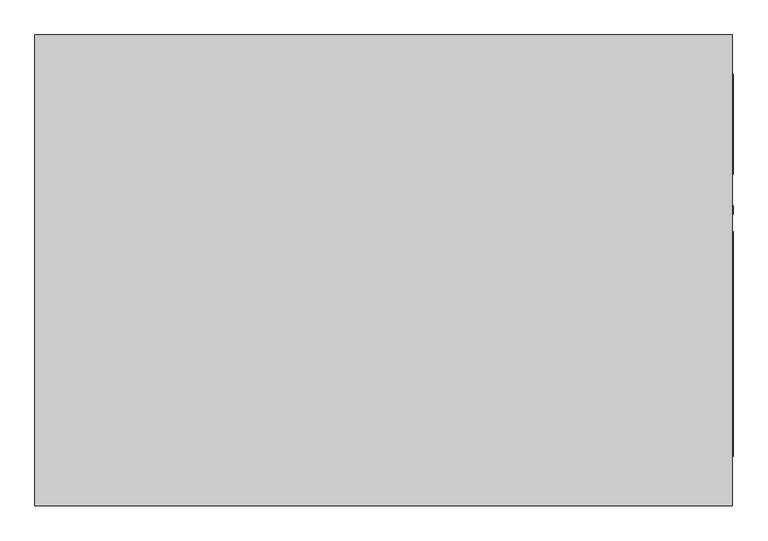
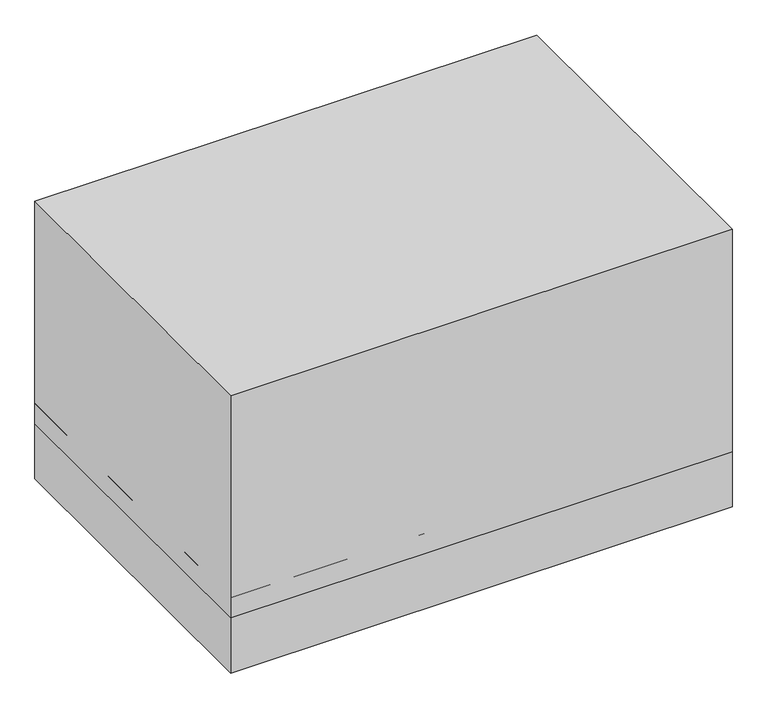
"""IFC4 building model written with IfcOpenShell, lengths in millimetres: proxy geometry, Carrier_48TC_Standard_Efficiency_Gas_Heat_Electric_Cooling_Packaged_Rooftop_Unit_3_to_15_nominal_tons : 7.5 ton 48TC**08."""

from ifc_helpers import new_model, si_unit, point, frame, frame_2d, origin, origin_with_axes, place, context, project, spatial, polyline, circle_curve, trimmed, segment, composite_curve, outline, extrude, source, transform, mapped, element, save
from ifc_brep_helpers import plane_surface, revolved_surface, advanced_brep


def mechanical_equipment_22992897(model_context):
    return source(origin(), model_context, "Body", "SolidModel", [
        extrude(outline(composite_curve([segment(trimmed(circle_curve(frame_2d((193.675, 438.15)), 13.2953125), [point((180.3796875, 438.15))], [point((206.9703125, 438.15))], False, "CARTESIAN"), True, "CONTINUOUS"), segment(trimmed(circle_curve(frame_2d((193.675, 438.15)), 13.2953125), [point((206.9703125, 438.15))], [point((180.3796875, 438.15))], False, "CARTESIAN"), True, "CONTINUOUS")], self_intersect=False)), frame((1119.1875, 0.0, 0.0), z_axis=(1.0, 0.0, 0.0), x_axis=(0.0, 1.0, 0.0)), (0.0, 0.0, 1.0), 3.175),
        advanced_brep(
        [(1119.1875, 755.65, 1308.1), (-1119.1875, 755.65, 1308.1), (-1119.1875, -755.65, 1308.1), (1119.1875, -755.65, 1308.1), (1119.1875, 755.65, 260.35), (1119.1875, -755.65, 260.35), (-1119.1875, -755.65, 260.35), (-1119.1875, 755.65, 260.35), (1036.6375, -596.9, 260.35), (1036.6375, 0.0, 260.35), (681.0375, 0.0, 260.35), (681.0375, -596.9, 260.35), (1036.6375, 590.55, 260.35), (112.7125, 590.55, 260.35), (112.7125, 269.875, 260.35), (1036.6375, 269.875, 260.35), (176.8078125, -107.95, 260.35), (150.2171875, -107.95, 260.35), (-355.6, -476.25, 260.35), (-377.825, -476.25, 260.35), (-344.4875, -349.25, 260.35), (-388.9375, -349.25, 260.35), (-344.4875, -298.45, 260.35), (-388.9375, -298.45, 260.35), (1036.6375, -596.9, 381.0), (681.0375, -596.9, 381.0), (681.0375, 0.0, 381.0), (1036.6375, 0.0, 381.0), (1036.6375, 590.55, 381.0), (1036.6375, 269.875, 381.0), (112.7125, 269.875, 381.0), (112.7125, 590.55, 381.0), (176.8078125, -107.95, 406.4), (150.2171875, -107.95, 406.4), (-355.6, -476.25, 406.4), (-377.825, -476.25, 406.4), (-344.4875, -349.25, 406.4), (-388.9375, -349.25, 406.4), (-344.4875, -298.45, 406.4), (-388.9375, -298.45, 406.4)],
        [
            (0, 1),
            (1, 2),
            (2, 3),
            (3, 0),
            (4, 5),
            (5, 6),
            (6, 7),
            (7, 4),
            (8, 9),
            (9, 10),
            (10, 11),
            (11, 8),
            (12, 13),
            (13, 14),
            (14, 15),
            (15, 12),
            (16, 17, circle_curve(frame((163.5125, -107.95, 260.35), z_axis=(0.0, 0.0, 1.0), x_axis=(-1.0, 0.0, 0.0)), 13.2953125)),
            (17, 16, circle_curve(frame((163.5125, -107.95, 260.35), z_axis=(0.0, 0.0, 1.0), x_axis=(-1.0, 0.0, 0.0)), 13.2953125)),
            (18, 19, circle_curve(frame((-366.7125, -476.25, 260.35), z_axis=(0.0, 0.0, 1.0), x_axis=(-1.0, 0.0, 0.0)), 11.1125)),
            (19, 18, circle_curve(frame((-366.7125, -476.25, 260.35), z_axis=(0.0, 0.0, 1.0), x_axis=(-1.0, 0.0, 0.0)), 11.1125)),
            (20, 21, circle_curve(frame((-366.7125, -349.25, 260.35), z_axis=(0.0, 0.0, 1.0), x_axis=(-1.0, 0.0, 0.0)), 22.225)),
            (21, 20, circle_curve(frame((-366.7125, -349.25, 260.35), z_axis=(0.0, 0.0, 1.0), x_axis=(-1.0, 0.0, 0.0)), 22.225)),
            (22, 23, circle_curve(frame((-366.7125, -298.45, 260.35), z_axis=(0.0, 0.0, 1.0), x_axis=(-1.0, 0.0, 0.0)), 22.225)),
            (23, 22, circle_curve(frame((-366.7125, -298.45, 260.35), z_axis=(0.0, 0.0, 1.0), x_axis=(-1.0, 0.0, 0.0)), 22.225)),
            (0, 4),
            (7, 1),
            (6, 2),
            (5, 3),
            (24, 25),
            (25, 26),
            (26, 27),
            (27, 24),
            (27, 9),
            (8, 24),
            (26, 10),
            (25, 11),
            (28, 29),
            (29, 30),
            (30, 31),
            (31, 28),
            (31, 13),
            (12, 28),
            (30, 14),
            (29, 15),
            (32, 33, circle_curve(frame((163.5125, -107.95, 406.4), z_axis=(0.0, 0.0, -1.0), x_axis=(-1.0, 0.0, 0.0)), 13.2953125)),
            (33, 32, circle_curve(frame((163.5125, -107.95, 406.4), z_axis=(0.0, 0.0, -1.0), x_axis=(-1.0, 0.0, 0.0)), 13.2953125)),
            (33, 17),
            (16, 32),
            (34, 35, circle_curve(frame((-366.7125, -476.25, 406.4), z_axis=(0.0, 0.0, -1.0), x_axis=(-1.0, 0.0, 0.0)), 11.1125)),
            (35, 34, circle_curve(frame((-366.7125, -476.25, 406.4), z_axis=(0.0, 0.0, -1.0), x_axis=(-1.0, 0.0, 0.0)), 11.1125)),
            (35, 19),
            (18, 34),
            (36, 37, circle_curve(frame((-366.7125, -349.25, 406.4), z_axis=(0.0, 0.0, -1.0), x_axis=(-1.0, 0.0, 0.0)), 22.225)),
            (37, 36, circle_curve(frame((-366.7125, -349.25, 406.4), z_axis=(0.0, 0.0, -1.0), x_axis=(-1.0, 0.0, 0.0)), 22.225)),
            (37, 21),
            (20, 36),
            (38, 39, circle_curve(frame((-366.7125, -298.45, 406.4), z_axis=(0.0, 0.0, -1.0), x_axis=(-1.0, 0.0, 0.0)), 22.225)),
            (39, 38, circle_curve(frame((-366.7125, -298.45, 406.4), z_axis=(0.0, 0.0, -1.0), x_axis=(-1.0, 0.0, 0.0)), 22.225)),
            (39, 23),
            (22, 38),
        ],
        [
            plane_surface(frame((-1119.1875, 755.65, 1308.1), z_axis=(0.0, 0.0, 1.0), x_axis=(-1.0, 0.0, 0.0))),
            plane_surface(frame((-1119.1875, 755.65, 260.35), z_axis=(0.0, 0.0, -1.0), x_axis=(1.0, 0.0, 0.0))),
            plane_surface(frame((1119.1875, 755.65, 1308.1), z_axis=(0.0, 1.0, 0.0), x_axis=(0.0, 0.0, -1.0))),
            plane_surface(frame((-1119.1875, 755.65, 1308.1), z_axis=(-1.0, 0.0, 0.0), x_axis=(0.0, 0.0, -1.0))),
            plane_surface(frame((-1119.1875, -755.65, 1308.1), z_axis=(0.0, -1.0, 0.0), x_axis=(0.0, 0.0, -1.0))),
            plane_surface(frame((1119.1875, -755.65, 1308.1), z_axis=(1.0, 0.0, 0.0), x_axis=(0.0, 0.0, -1.0))),
            plane_surface(frame((1036.6375, -596.9, 381.0), z_axis=(0.0, 0.0, -1.0), x_axis=(0.0, 1.0, 0.0))),
            plane_surface(frame((1036.6375, -596.9, 381.0), z_axis=(-1.0, 0.0, 0.0), x_axis=(0.0, 0.0, -1.0))),
            plane_surface(frame((1036.6375, 0.0, 381.0), z_axis=(0.0, -1.0, 0.0), x_axis=(0.0, 0.0, -1.0))),
            plane_surface(frame((681.0375, 0.0, 381.0), z_axis=(1.0, 0.0, 0.0), x_axis=(0.0, 0.0, -1.0))),
            plane_surface(frame((681.0375, -596.9, 381.0), z_axis=(0.0, 1.0, 0.0), x_axis=(0.0, 0.0, -1.0))),
            plane_surface(frame((112.7125, 590.55, 381.0), z_axis=(0.0, 0.0, -1.0), x_axis=(-1.0, 0.0, 0.0))),
            plane_surface(frame((1036.6375, 590.55, 381.0), z_axis=(0.0, -1.0, 0.0), x_axis=(0.0, 0.0, -1.0))),
            plane_surface(frame((112.7125, 590.55, 381.0), z_axis=(1.0, 0.0, 0.0), x_axis=(0.0, 0.0, -1.0))),
            plane_surface(frame((112.7125, 269.875, 381.0), z_axis=(0.0, 1.0, 0.0), x_axis=(0.0, 0.0, -1.0))),
            plane_surface(frame((1036.6375, 269.875, 381.0), z_axis=(-1.0, 0.0, 0.0), x_axis=(0.0, 0.0, -1.0))),
            plane_surface(frame((150.2171875, -107.95, 406.4), z_axis=(0.0, 0.0, -1.0), x_axis=(0.0, -1.0, 0.0))),
            revolved_surface(polyline([(150.2171875, -107.95, 406.4), (150.2171875, -107.95, 260.35)]), (163.5125, -107.95, 0.0), (0.0, 0.0, 1.0)),
            plane_surface(frame((-377.825, -476.25, 406.4), z_axis=(0.0, 0.0, -1.0), x_axis=(0.0, -1.0, 0.0))),
            revolved_surface(polyline([(-377.825, -476.25, 406.4), (-377.825, -476.25, 260.35)]), (-366.7125, -476.25, 0.0), (0.0, 0.0, 1.0)),
            plane_surface(frame((-388.9375, -349.25, 406.4), z_axis=(0.0, 0.0, -1.0), x_axis=(0.0, -1.0, 0.0))),
            revolved_surface(polyline([(-388.9375, -349.25, 406.4), (-388.9375, -349.25, 260.35)]), (-366.7125, -349.25, 0.0), (0.0, 0.0, 1.0)),
            plane_surface(frame((-388.9375, -298.45, 406.4), z_axis=(0.0, 0.0, -1.0), x_axis=(0.0, -1.0, 0.0))),
            revolved_surface(polyline([(-388.9375, -298.45, 406.4), (-388.9375, -298.45, 260.35)]), (-366.7125, -298.45, 0.0), (0.0, 0.0, 1.0)),
        ],
        [
            (0, [[1, 2, 3, 4]]),
            (1, [[5, 6, 7, 8], [9, 10, 11, 12], [13, 14, 15, 16], [17, 18], [19, 20], [21, 22], [23, 24]]),
            (2, [[-1, 25, -8, 26]]),
            (3, [[-2, -26, -7, 27]]),
            (4, [[-3, -27, -6, 28]]),
            (5, [[-4, -28, -5, -25]]),
            (6, [[29, 30, 31, 32]]),
            (7, [[-32, 33, -9, 34]]),
            (8, [[-31, 35, -10, -33]]),
            (9, [[-30, 36, -11, -35]]),
            (10, [[-29, -34, -12, -36]]),
            (11, [[37, 38, 39, 40]]),
            (12, [[-40, 41, -13, 42]]),
            (13, [[-39, 43, -14, -41]]),
            (14, [[-38, 44, -15, -43]]),
            (15, [[-37, -42, -16, -44]]),
            (16, [[45, 46]]),
            (17, [[-46, 47, -17, 48]]),
            (17, [[-45, -48, -18, -47]]),
            (18, [[49, 50]]),
            (19, [[-50, 51, -19, 52]]),
            (19, [[-49, -52, -20, -51]]),
            (20, [[53, 54]]),
            (21, [[-54, 55, -21, 56]]),
            (21, [[-53, -56, -22, -55]]),
            (22, [[57, 58]]),
            (23, [[-58, 59, -23, 60]]),
            (23, [[-57, -60, -24, -59]]),
        ],
    ),
        extrude(outline(polyline([(1119.1875, 755.65), (1119.1875, -755.65), (-1119.1875, -755.65), (-1119.1875, 755.65), (1119.1875, 755.65)]), holes=[polyline([(1036.6375, 590.55), (112.7125, 590.55), (112.7125, 269.875), (1036.6375, 269.875), (1036.6375, 590.55)]), polyline([(1036.6375, -596.9), (1036.6375, 0.0), (681.0375, 0.0), (681.0375, -596.9), (1036.6375, -596.9)]), composite_curve([segment(trimmed(circle_curve(frame_2d((163.5125, -107.95)), 13.2953125), [point((176.8078125, -107.95))], [point((150.2171875, -107.95))], True, "CARTESIAN"), True, "CONTINUOUS"), segment(trimmed(circle_curve(frame_2d((163.5125, -107.95)), 13.2953125), [point((150.2171875, -107.95))], [point((176.8078125, -107.95))], True, "CARTESIAN"), True, "CONTINUOUS")], self_intersect=False), composite_curve([segment(trimmed(circle_curve(frame_2d((-366.7125, -476.25)), 11.1125), [point((-355.6, -476.25))], [point((-377.825, -476.25))], True, "CARTESIAN"), True, "CONTINUOUS"), segment(trimmed(circle_curve(frame_2d((-366.7125, -476.25)), 11.1125), [point((-377.825, -476.25))], [point((-355.6, -476.25))], True, "CARTESIAN"), True, "CONTINUOUS")], self_intersect=False), composite_curve([segment(trimmed(circle_curve(frame_2d((-366.7125, -349.25)), 22.225), [point((-344.4875, -349.25))], [point((-388.9375, -349.25))], True, "CARTESIAN"), True, "CONTINUOUS"), segment(trimmed(circle_curve(frame_2d((-366.7125, -349.25)), 22.225), [point((-388.9375, -349.25))], [point((-344.4875, -349.25))], True, "CARTESIAN"), True, "CONTINUOUS")], self_intersect=False), composite_curve([segment(trimmed(circle_curve(frame_2d((-366.7125, -298.45)), 22.225), [point((-344.4875, -298.45))], [point((-388.9375, -298.45))], True, "CARTESIAN"), True, "CONTINUOUS"), segment(trimmed(circle_curve(frame_2d((-366.7125, -298.45)), 22.225), [point((-388.9375, -298.45))], [point((-344.4875, -298.45))], True, "CARTESIAN"), True, "CONTINUOUS")], self_intersect=False)]), origin_with_axes(), (0.0, 0.0, 1.0), 355.6),
        extrude(outline(polyline([(1122.3625, 628.65), (1122.3625, 307.975), (1119.1875, 307.975), (1119.1875, 628.65), (1122.3625, 628.65)])), frame((0.0, 0.0, 406.4), z_axis=(0.0, 0.0, 1.0), x_axis=(1.0, 0.0, 0.0)), (0.0, 0.0, 1.0), 857.25),
        extrude(outline(polyline([(1122.3625, 123.825), (1122.3625, -596.9), (1119.1875, -596.9), (1119.1875, 123.825), (1122.3625, 123.825)])), frame((0.0, 0.0, 406.4), z_axis=(0.0, 0.0, 1.0), x_axis=(1.0, 0.0, 0.0)), (0.0, 0.0, 1.0), 352.425),
    ])


if __name__ == "__main__":
    model = new_model("IFC4")
    model_context = context("Model", 3, world=origin())
    ifc_project = project(units=[si_unit("LENGTHUNIT", "METRE", prefix="MILLI")], contexts=[model_context])
    site = spatial("IfcSite", under=ifc_project)
    building = spatial("IfcBuilding", under=site)
    placement = place(None, origin())
    mechanical_equipment_shape = mechanical_equipment_22992897(model_context)
    element("IfcBuildingElementProxy", 1, Name="Carrier_48TC_Standard_Efficiency_Gas_Heat_Electric_Cooling_Packaged_Rooftop_Unit_3_to_15_nominal_tons : 7.5 ton 48TC**08", ObjectType="Carrier_48TC_Standard_Efficiency_Gas_Heat_Electric_Cooling_Packaged_Rooftop_Unit_3_to_15_nominal_tons : 7.5 ton 48TC**08", at=placement, inside=building, context=model_context, shape_type="MappedRepresentation", body=[
        mapped(mechanical_equipment_shape, transform((0.0, 0.0, 0.0), x_axis=(1.0, 0.0, 0.0), y_axis=(0.0, 1.0, 0.0), z_axis=(0.0, 0.0, 1.0))),
    ])
    save(model, "model.ifc")

# Revit data of these elements
# Type "Carrier_48TC_Standard_Efficiency_Gas_Heat_Electric_Cooling_Packaged_Rooftop_Unit_3_to_15_nominal_tons : 7.5 ton 48TC**08"
#   URL = "www.Carrier.com"
#   Model = "48TC"
#   Manufacturer = "Carrier"
#   Disclaimer = "Manufacturer reserves the right to change, at any time, specifications and designs without notice and without obligation.  Please verify critical parameters with local Carrier commercial sales office."
#   knockout thickness = 0' - 0 1/16"
#   Voltage = 0 V
#   Version = 1
#   TTBY3 = 0' - 11"
#   TTBY2 = 1' - 4"
#   TTBY1 = 1' - 6"
#   TTBX = 2' - 5 5/8"
#   TTBPowerR = 0' - 0 7/8"
#   TTBGasR = 0' - 0 7/8"
#   SSSZ = 0' - 5 3/4"
#   SSSY = 0' - 6 1/4"
#   SSSW = 2' - 4 3/8"
#   SSSH = 1' - 1 7/8"
#   SSRZ = 0' - 5 3/4"
#   SSRY = 0' - 5"
#   SSRW = 1' - 0 5/8"
#   SSRH = 2' - 9 3/4"
#   SEER = 0
#   Right clearance = 3' - 0"
#   PWRZ = 2' - 3 7/8"
#   PWRY = 0' - 4 5/8"
#   PWRR = 0' - 1 1/4"
#   ODF2X = 1' - 0"
#   ODF1Y = 0' - 11"
#   ODF1X = 2' - 1"
#   ODF1R = 0' - 10"
#   MOCP = 0 A
#   MCA = 0 A
#   Left clearance = 4' - 0"
#   IEER = 11.7
#   Front clearance = 4' - 0"
#   Fan Z = 4' - 3 1/2"
#   Width = 4' - 11 1/2"
#   Length = 7' - 4 1/8"
#   Height = 3' - 5 1/4"
#   EER = 11
#   DSSY = 0' - 6 1/4"
#   DSSX = 0' - 3 1/4"
#   DSSW = 1' - 2"
#   DSSH = 2' - 4 3/4"
#   DSRY = 0' - 6 1/2"
#   DSRX = 0' - 3 1/4"
#   DSRW = 3' - 0 3/8"
#   DSRH = 1' - 0 5/8"
#   DRNZ = 0' - 7"
#   DRNY = 3' - 1 3/8"
#   DRNR = 0' - 0 67/128"
#   Curb Z = 1' - 2"
#   CFM (nominal) = 0 CFM
#   Back clearance = 3' - 0"
#   Alt Condensate Drain = 0' - 0 67/128"
#   AccypwrR = 0' - 0 7/16"
#   ACY = 2' - 1 1/2"
#   ACX = 3' - 1 5/8"
#   Gas [instance default] = yes
#   Fan 2 on = yes
#   Curb_1SLAB_2ROOFCURB_3SNOWCURB = 2
#   Fan 3 on = no
#   Unit material = SINGLE-PACKAGED ROOFTOP UNITS
#   Curb material = Curb paint
# Element 1 (IfcBuildingElementProxy, "Carrier_48TC_Standard_Efficiency_Gas_Heat_Electric_Cooling_Packaged_Rooftop_Unit_3_to_15_nominal_tons : 7.5 ton 48TC**08")
#   Materials on its faces: "SINGLE-PACKAGED ROOFTOP UNITS", "Curb paint", "Mech"
# Materials
#   "SINGLE-PACKAGED ROOFTOP UNITS": class "Miscellaneous", colour RGB 201 201 201, transparency 0, Cost = 0
#   "Curb paint": class "Miscellaneous", colour RGB 189 187 185, transparency 0
#   "Mech": class "Miscellaneous", colour RGB 235 237 235, transparency 0, Cost = 0
